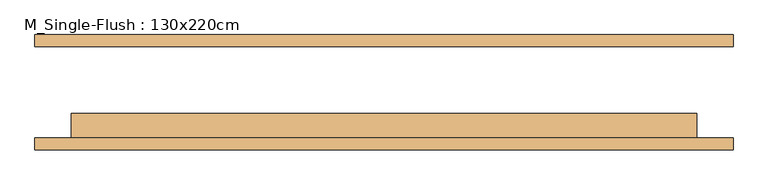
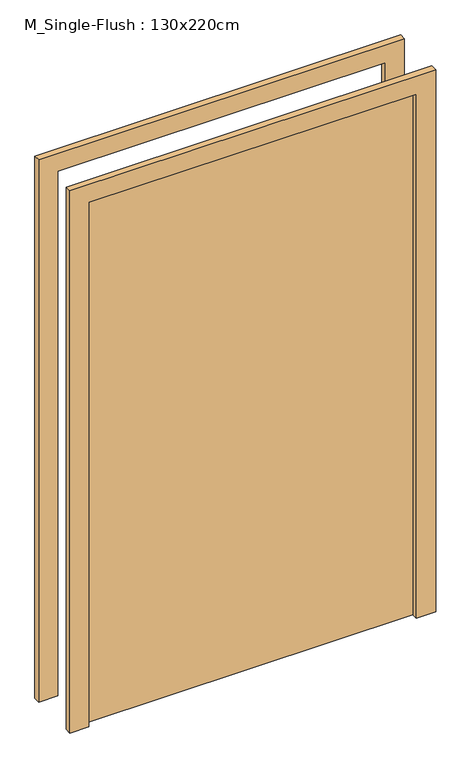
"""IFC4 building model written with IfcOpenShell, lengths in millimetres: door geometry, M_Single-Flush : 130x220cm."""

from ifc_helpers import new_model, si_unit, frame, origin, origin_with_axes, place, context, project, spatial, polyline, outline, extrude, source, transform, mapped, element, save


def m_single_flush_130x220cm_6f91bfee(model_context):
    return source(origin(), model_context, "Body", "SweptSolid", [
        extrude(outline(polyline([(2276.0, -726.0), (0.0, -726.0), (0.0, -650.0), (2200.0, -650.0), (2200.0, 650.0), (0.0, 650.0), (0.0, 726.0), (2276.0, 726.0), (2276.0, -726.0)])), frame((0.0, -120.0, 0.0), z_axis=(0.0, 1.0, 0.0), x_axis=(0.0, 0.0, 1.0)), (0.0, 0.0, 1.0), 25.0),
        extrude(outline(polyline([(2276.0, 726.0), (2276.0, -726.0), (0.0, -726.0), (0.0, -650.0), (2200.0, -650.0), (2200.0, 650.0), (0.0, 650.0), (0.0, 726.0), (2276.0, 726.0)])), frame((0.0, 95.0, 0.0), z_axis=(0.0, 1.0, 0.0), x_axis=(0.0, 0.0, 1.0)), (0.0, 0.0, 1.0), 25.0),
        extrude(outline(polyline([(650.0, -44.0), (650.0, -95.0), (-650.0, -95.0), (-650.0, -44.0), (650.0, -44.0)])), origin_with_axes(), (0.0, 0.0, 1.0), 2200.0),
    ])


if __name__ == "__main__":
    model = new_model("IFC4")
    model_context = context("Model", 3, world=origin())
    ifc_project = project(units=[si_unit("LENGTHUNIT", "METRE", prefix="MILLI")], contexts=[model_context])
    site = spatial("IfcSite", under=ifc_project)
    building = spatial("IfcBuilding", under=site)
    placement = place(None, origin())
    m_single_flush_130x220cm_shape = m_single_flush_130x220cm_6f91bfee(model_context)
    element("IfcDoor", 1, ObjectType="M_Single-Flush : 130x220cm", at=placement, inside=building, context=model_context, shape_type="MappedRepresentation", body=[
        mapped(m_single_flush_130x220cm_shape, transform((0.0, 0.0, 0.0), x_axis=(1.0, 0.0, 0.0), y_axis=(0.0, 1.0, 0.0), z_axis=(0.0, 0.0, 1.0))),
    ])
    save(model, "model.ifc")

# Revit data of these elements
# Type "M_Single-Flush : 130x220cm"
#   Type Mark = "46"
#   Construction Type Id = "MDOOR"
#   Analytic Construction = "Metal"
#   Thickness = 5.10 cm
#   Heat Transfer Coefficient (U) = 3.7021 W/(m²·K)
#   Height = 220.00 cm
#   Trim Projection Ext = 2.50 cm
#   Trim Projection Int = 2.50 cm
#   Trim Width = 7.60 cm
#   Width = 130.00 cm
#   Define Thermal Properties by = 1
#   Door Material = Door - Panel
#   Frame Material = Door - Frame
#   Visual Light Transmittance = 0
#   Solar Heat Gain Coefficient = 0
#   Function = (empty or 0)
#   Wall Closure = (empty or 0)
# Element 1 (IfcDoor, "M_Single-Flush : 130x220cm")
#   Materials on its faces: "Door - Frame", "Door - Panel"
# Materials
#   "Door - Panel": class "Wood", colour RGB 210 159 95, transparency 0, Cost = 0
#   "Door - Frame": class "Miscellaneous", colour RGB 118 70 51, transparency 0, Cost = 0
